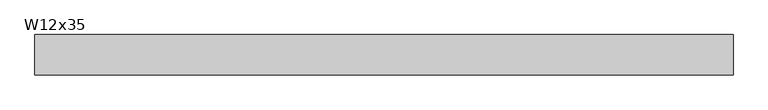
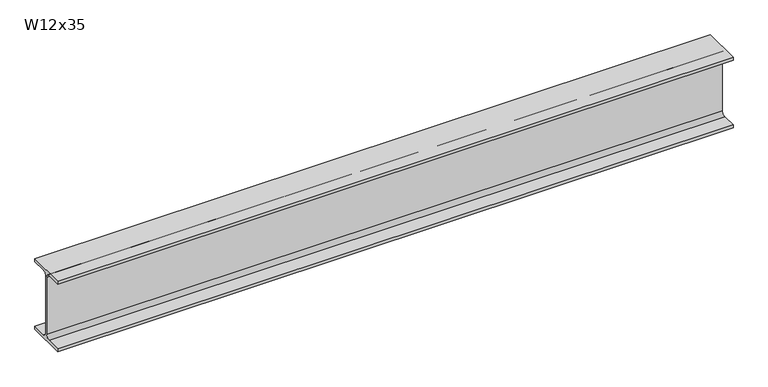
"""IFC4 building model written with IfcOpenShell, lengths in millimetres: beam geometry, RME W-Wide Flange : W12x35."""

from ifc_helpers import new_model, si_unit, point, frame, frame_2d, origin, place, context, project, spatial, polyline, circle_curve, trimmed, segment, composite_curve, outline, extrude, source, transform, mapped, element, save


def w12x35_037dfd65(model_context):
    return source(origin(), model_context, "Body", "SweptSolid", [
        extrude(outline(composite_curve([segment(polyline([(83.312, -145.542), (83.312, -158.75), (-83.312, -158.75), (-83.312, -145.542), (-20.7645, -145.542)]), True, "CONTINUOUS"), segment(trimmed(circle_curve(frame_2d((-20.7645, -128.5875)), 16.9545), [point((-20.7645, -145.542))], [point((-3.81, -128.5875))], True, "CARTESIAN"), True, "CONTINUOUS"), segment(polyline([(-3.81, -128.5875), (-3.81, 128.5875)]), True, "CONTINUOUS"), segment(trimmed(circle_curve(frame_2d((-20.7645, 128.5875)), 16.9545), [point((-3.81, 128.5875))], [point((-20.7645, 145.542))], True, "CARTESIAN"), True, "CONTINUOUS"), segment(polyline([(-20.7645, 145.542), (-83.312, 145.542), (-83.312, 158.75), (83.312, 158.75), (83.312, 145.542), (20.7645, 145.542)]), True, "CONTINUOUS"), segment(trimmed(circle_curve(frame_2d((20.7645, 128.5875)), 16.9545), [point((20.7645, 145.542))], [point((3.81, 128.5875))], True, "CARTESIAN"), True, "CONTINUOUS"), segment(polyline([(3.81, 128.5875), (3.81, -128.5875)]), True, "CONTINUOUS"), segment(trimmed(circle_curve(frame_2d((20.7645, -128.5875)), 16.9545), [point((3.81, -128.5875))], [point((20.7645, -145.542))], True, "CARTESIAN"), True, "CONTINUOUS"), segment(polyline([(20.7645, -145.542), (83.312, -145.542)]), True, "CONTINUOUS")], self_intersect=False)), frame((-1441.028357, 0.0, 0.0), z_axis=(1.0, 0.0, 0.0), x_axis=(0.0, 1.0, 0.0)), (0.0, 0.0, 1.0), 2875.5494132),
    ])


if __name__ == "__main__":
    model = new_model("IFC4")
    model_context = context("Model", 3, world=origin())
    ifc_project = project(units=[si_unit("LENGTHUNIT", "METRE", prefix="MILLI")], contexts=[model_context])
    site = spatial("IfcSite", under=ifc_project)
    building = spatial("IfcBuilding", under=site)
    placement = place(None, origin())
    w12x35_shape = w12x35_037dfd65(model_context)
    element("IfcBeam", 1, ObjectType="RME W-Wide Flange : W12x35", at=placement, inside=building, context=model_context, shape_type="MappedRepresentation", body=[
        mapped(w12x35_shape, transform((0.0, 0.0, 0.0), x_axis=(1.0, 0.0, 0.0), y_axis=(0.0, 1.0, 0.0), z_axis=(0.0, 0.0, 1.0))),
    ])
    save(model, "model.ifc")

# Revit data of these elements
# Type "RME W-Wide Flange : W12x35"
#   WELD P [instance default] = ""
#   WELD LE [instance default] = ""
#   WELD D [instance default] = ""
#   TOP SECTION SIZE [instance default] = ""
#   TOP SECTION LENGTH [instance default] = ""
#   REMARKS [instance default] = ""
#   REINF TYPE [instance default] = ""
#   Nominal Size = "W24"
#   End Bearing Capacity [instance default] = ""
#   BOT SECTION SIZE [instance default] = ""
#   BOT SECTION LENGTH [instance default] = ""
#   Assembly Code = "B10"
#   W = 35
#   Start Extension Calculation [instance default] = 10' - 0"
#   Start Extension [instance default] = -0' - 0 1/2"
#   End Extension Calculation [instance default] = 10' - 0"
#   End Extension [instance default] = -0' - 0 1/2"
#   Length [instance default] = 5' - 0"
#   bf = 0' - 6.56"
#   d = 1' - 0 1/2"
#   k = 0' - 1 3/16"
#   k2 = 0' - 0.6675"
#   tf = 0' - 0.52"
#   tw = 0' - 0.3"
#   A = 0.0715278 SF
#   Structural Material [instance default] = Metal - Steel - ASTM A992
# Element 1 (IfcBeam, "RME W-Wide Flange : W12x35")
#   Length = 10' - 1.02542"
#   Materials on its faces: "Metal - Steel - ASTM A992"
# Materials
#   "Metal - Steel - ASTM A992": class "Metal", colour RGB 255 128 0, transparency 0
